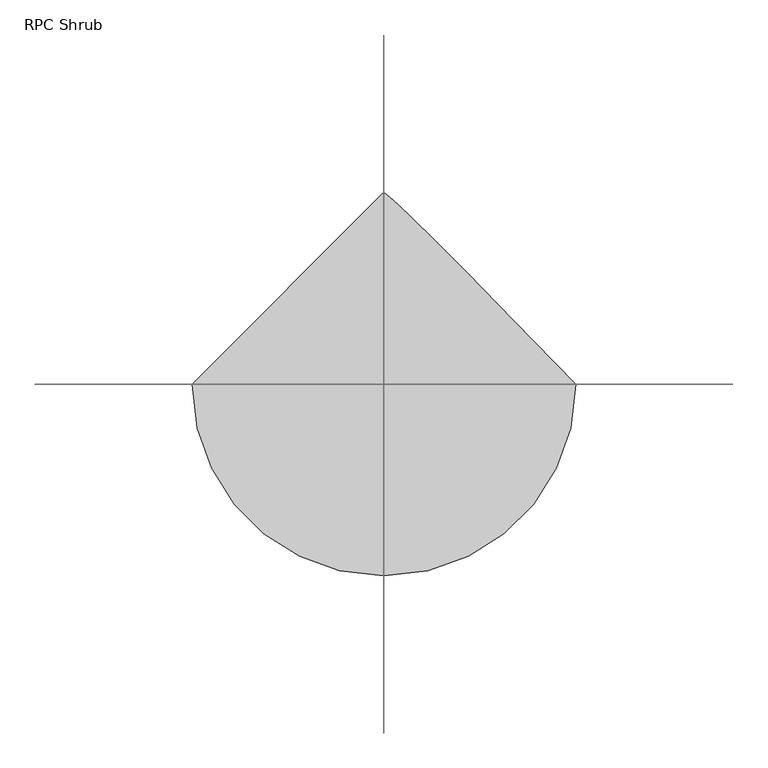
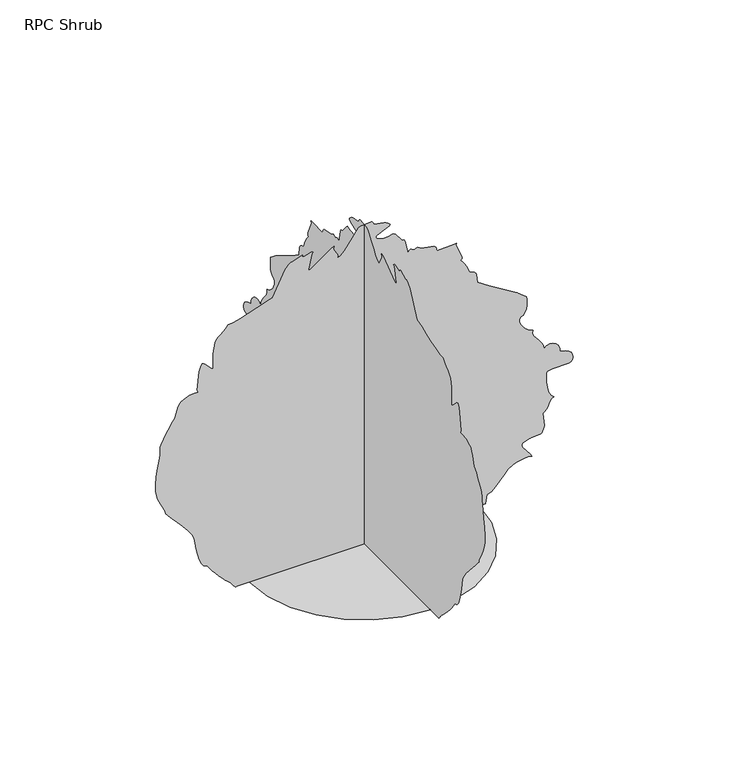
"""IFC4 building model written with IfcOpenShell, lengths in millimetres: geographic element geometry, RPC Shrub."""

from ifc_helpers import new_model, si_unit, origin, place, context, project, spatial, triangles, source, transform, mapped, element, save


def rpc_shrub_5c4a15e9(model_context):
    return source(origin(), model_context, "Body", "Tessellation", [
        triangles([(-310.4009663, 0.0, 0.0), (-302.1967432, -71.1236111, 0.0), (-278.8261857, -136.4392555, 0.0), (-242.1615087, -194.0757083, 0.0), (-194.0757083, -242.1615087, 0.0), (-136.4392555, -278.8261857, 0.0), (-71.1236111, -302.1967432, 0.0), (1.36e-05, -310.4009663, 0.0), (71.1236111, -302.1967432, 0.0), (136.4392555, -278.8261857, 0.0), (194.0757083, -242.1615087, 0.0), (242.1615087, -194.0757083, 0.0), (278.8261857, -136.4392555, 0.0), (302.1967432, -71.1236111, 0.0), (310.4009663, 2.71e-05, 0.0), (209.5283262, 103.4718092, 0.0), (134.7455816, 179.6535872, 0.0), (81.7052599, 233.0934394, 0.0), (46.0591254, 268.3410517, 0.0), (23.45852, 289.9412231, 0.0), (9.5549798, 302.4456561, 0.0), (-4.07e-05, 310.4009663, 0.0), (-352.7554667, 2.15e-05, 4.3495503), (-355.9965117, 2.13e-05, 8.4826161), (-359.0826241, 2.1e-05, 12.3234041), (-362.0188548, 2.08e-05, 15.7959676), (-364.8077834, 2.07e-05, 18.8245652), (-367.457004, 2.05e-05, 21.3332227), (-369.9665528, 2.04e-05, 23.2460988), (-375.8161594, 2.01e-05, 28.5320975), (-383.5606359, 1.96e-05, 36.3306653), (-392.4582396, 1.9e-05, 45.9079945), (-401.7775108, 1.84e-05, 56.5300297), (-410.7742001, 1.78e-05, 67.463215), (-418.7091808, 1.71e-05, 77.9737471), (-424.8483773, 1.66e-05, 87.3278091), (-434.3200376, 1.64e-05, 90.3102761), (-441.518399, 1.59e-05, 99.1873323), (-446.9133459, 1.51e-05, 112.4136326), (-450.9672046, 1.41e-05, 128.4448579), (-454.1523663, 1.31e-05, 145.7354086), (-456.9311211, 1.21e-05, 162.7404662), (-459.7733894, 1.12e-05, 177.9152122), (-465.8821009, 1.05e-05, 189.8085088), (-476.9463238, 9.6e-06, 205.0848474), (-490.9620744, 8.5e-06, 222.0754346), (-505.927767, 7.5e-06, 239.1112225), (-519.8393452, 6.6e-06, 254.5234358), (-530.6927888, 5.9e-06, 266.6443348), (-536.4840051, 5.5e-06, 273.804599), (-537.980062, 5.1e-06, 279.9056801), (-541.2769901, 4.6e-06, 287.7695352), (-545.6533945, 4.1e-06, 296.6874683), (-550.3904963, 3.6e-06, 305.9584685), (-554.7669371, 3e-06, 314.8764198), (-558.0638288, 2.6e-06, 322.7377496), (-559.5599221, 2.2e-06, 328.8413741), (-564.0633173, 1.1e-06, 346.2505222), (-564.6424607, -1e-07, 367.0963428), (-562.5393188, -1.4e-06, 389.5906094), (-558.9909525, -2.8e-06, 411.9375375), (-555.2393646, -4e-06, 432.3439227), (-552.5215799, -5e-06, 449.0164879), (-552.0770576, -5.6e-06, 460.1619922), (-551.4522048, -6.2e-06, 469.7809908), (-548.1832546, -6.8e-06, 479.8495623), (-543.0422894, -7.4e-06, 490.1772022), (-536.8090942, -8.1e-06, 500.5785295), (-530.2609838, -8.7e-06, 510.8553732), (-524.1776705, -9.2e-06, 520.822352), (-519.3338891, -9.8e-06, 530.2863819), (-514.6958364, -1.01e-05, 534.5764544), (-511.1779552, -1.05e-05, 541.7037083), (-508.3280565, -1.1e-05, 550.5352913), (-505.7042341, -1.16e-05, 559.930757), (-502.8569152, -1.21e-05, 568.7597966), (-499.3364542, -1.25e-05, 575.8870505), (-494.6984015, -1.28e-05, 580.1796301), (-488.7141738, -1.3e-05, 583.3724221), (-483.0575787, -1.32e-05, 586.1308657), (-477.4467293, -1.33e-05, 588.3914835), (-471.5996298, -1.34e-05, 590.0856388), (-465.2318499, -1.35e-05, 591.1448401), (-458.0563431, -1.35e-05, 591.5029578), (-449.7962731, -1.35e-05, 591.0940438), (-452.0898831, -1.38e-05, 597.7844058), (-446.8498687, -1.69e-05, 648.1323137), (-442.8239516, -1.75e-05, 659.7223766), (-438.0639951, -1.8e-05, 668.1551468), (-434.5155925, -1.8e-05, 667.6064884), (-430.9748566, -1.79e-05, 665.0360058), (-414.5257879, -1.68e-05, 647.428723), (-409.2578319, -1.66e-05, 644.4162615), (-408.9962199, -1.74e-05, 657.4007887), (-409.1181238, -1.79e-05, 666.2653639), (-409.3213454, -1.83e-05, 672.7017443), (-409.3035413, -1.87e-05, 678.4040852), (-408.7625133, -1.91e-05, 685.0639257), (-407.3934834, -1.96e-05, 694.3755667), (-404.8915649, -2.04e-05, 708.0306198), (-403.2913719, -2.1e-05, 717.4769182), (-399.8064829, -2.14e-05, 724.3451036), (-394.8255369, -2.17e-05, 729.6460882), (-388.7295427, -2.2e-05, 734.3907841), (-381.9096102, -2.23e-05, 739.5952629), (-374.7468206, -2.27e-05, 746.2703642), (-367.6271971, -2.33e-05, 755.4296162), (-354.5182589, -2.33e-05, 756.2449734), (-335.3386883, -2.36e-05, 761.043009), (-312.9155657, -2.4e-05, 768.2718555), (-290.0885433, -2.45e-05, 776.3821163), (-269.6872632, -2.49e-05, 783.819235), (-254.5437653, -2.53e-05, 789.0313442), (-247.4939957, -2.53e-05, 790.4715179), (-213.6794536, -2.94e-05, 858.769602), (-205.2583288, -3e-05, 869.5493946), (-197.3670409, -3.03e-05, 874.0807314), (-193.2331907, -3.03e-05, 873.8495682), (-168.7295447, -3.09e-05, 884.1188541), (-166.460806, -3.09e-05, 883.4558859), (-168.0742249, -3.06e-05, 879.0896553), (-161.877383, -3.06e-05, 879.3893463), (-144.3734641, -3.09e-05, 884.8376329), (-141.0938133, -3.09e-05, 884.1543898), (-137.9627544, -3.07e-05, 881.4086271), (-140.7920603, -3.07e-05, 880.4332506), (-150.2901451, -2.82e-05, 838.0508085), (-150.4359393, -2.79e-05, 834.0097034), (-142.0369153, -2.81e-05, 837.3624784), (-89.9201382, -3.04e-05, 875.4065952), (-81.5211142, -3.06e-05, 878.7594429), (-83.236371, -3.02e-05, 872.9860308), (-82.0336828, -2.99e-05, 867.6621552), (-72.5891921, -2.9e-05, 852.5922901), (-71.3862495, -2.87e-05, 847.2684872), (-73.1015109, -2.84e-05, 841.495075), (-63.556186, -2.86e-05, 845.6047806), (-53.0855361, -2.92e-05, 856.2092932), (-42.3674857, -3.01e-05, 870.5983858), (-32.0797166, -3.1e-05, 886.0492596), (-22.9007347, -3.19e-05, 899.8541582), (-15.50783, -3.24e-05, 909.2952971), (-10.5790577, -3.25e-05, 911.6575075), (18.9106201, -3.27e-05, 914.4007267), (21.5322068, -3.27e-05, 913.1789989), (23.8564858, -3.25e-05, 909.8845779), (26.6850082, -3.21e-05, 903.8622711), (53.36646, -3.19e-05, 899.8287237), (58.7731068, -3.17e-05, 897.4639698), (63.9669031, -3.15e-05, 893.9232702), (69.0938976, -3.12e-05, 888.8939987), (68.0601171, -3.1e-05, 885.5234196), (63.3263127, -3.08e-05, 882.1706446), (34.7215748, -3.01e-05, 870.0904226), (31.9859905, -2.99e-05, 867.6900604), (32.133565, -2.97e-05, 863.7226427), (35.5686638, -2.95e-05, 860.1538925), (41.5277613, -2.93e-05, 857.2862623), (49.2473392, -2.92e-05, 855.4244574), (57.9630999, -2.92e-05, 854.8808859), (66.9122902, -2.92e-05, 855.9553116), (75.3308715, -2.94e-05, 858.9575993), (79.5358429, -2.94e-05, 858.9905914), (84.1909094, -2.92e-05, 855.1374109), (99.0570351, -2.8e-05, 835.8054514), (103.7123468, -2.78e-05, 831.9522709), (107.9173227, -2.78e-05, 831.9827196), (110.5566329, -2.75e-05, 826.9687815), (117.7400153, -2.54e-05, 791.6018269), (122.069702, -2.57e-05, 796.2169521), (125.2845857, -2.58e-05, 797.6521116), (127.9442162, -2.57e-05, 797.0729319), (133.8415943, -2.56e-05, 794.512623), (138.1999856, -2.56e-05, 794.8580961), (144.2457012, -2.58e-05, 797.8374928), (154.0983702, -2.54e-05, 791.6500797), (188.4892397, -2.5e-05, 784.7844378), (193.5639118, -2.47e-05, 779.5723286), (196.3218285, -2.41e-05, 769.7729994), (243.3426139, -2.42e-05, 771.0379658), (249.3334547, -2.43e-05, 772.2673239), (247.7520468, -2.39e-05, 766.8596598), (263.6852313, -2.17e-05, 729.0644377), (264.3888039, -2.13e-05, 722.3968941), (260.2486133, -2.11e-05, 719.5673429), (264.4396183, -2.09e-05, 715.6404751), (268.5899827, -2.05e-05, 710.080422), (272.58794, -2.02e-05, 703.4306826), (276.3268288, -1.97e-05, 696.2399878), (279.6948645, -1.93e-05, 689.0492203), (282.5828423, -1.89e-05, 682.4020243), (284.8815392, -1.86e-05, 676.8470581), (292.1535699, -1.84e-05, 674.5203833), (297.5205933, -1.82e-05, 671.6629269), (301.2772681, -1.8e-05, 668.0231054), (303.7181983, -1.78e-05, 663.3520243), (306.0880391, -1.64e-05, 640.6748474), (337.5484735, -1.51e-05, 619.285528), (412.8366832, -1.23e-05, 572.7882208), (438.1198783, -1.12e-05, 553.4791523), (439.8826341, -1.08e-05, 546.9589471), (439.9893136, -9.7e-06, 528.3128105), (438.1224217, -9.1e-06, 518.4956772), (434.833124, -8.6e-06, 509.8850836), (430.0172479, -8.2e-06, 503.634157), (423.57073, -8.1e-06, 500.8960247), (419.6083265, -7.7e-06, 495.2673712), (419.9613936, -7.3e-06, 487.2053996), (423.7561475, -6.7e-06, 477.8835849), (430.1112465, -6.1e-06, 468.4703513), (438.1503633, -5.6e-06, 460.136594), (446.9946273, -5.3e-06, 454.0533171), (455.7652765, -5.1e-06, 451.3913793), (454.5663671, -4.6e-06, 443.4767461), (457.9420332, -4.1e-06, 435.1353584), (464.2260246, -3.6e-06, 426.3952306), (471.7495116, -3.1e-06, 417.2791446), (478.8462805, -2.5e-06, 407.8151147), (483.8449943, -1.9e-06, 398.025923), (485.0794393, -1.3e-06, 387.9344968), (492.6181506, -1.7e-06, 394.3632468), (501.3405107, -1.8e-06, 396.5095548), (510.2914905, -1.8e-06, 394.9982735), (518.5109379, -1.5e-06, 390.4541831), (525.0463675, -1.1e-06, 383.5047526), (528.9401705, -5e-07, 374.7773057), (529.2322675, 0.0, 364.8966951), (543.28359, 2e-07, 361.6200783), (553.2505325, 5e-07, 356.9591709), (559.7300789, 8e-07, 351.3864369), (563.3267344, 1.2e-06, 345.3742312), (564.6424607, 1.5e-06, 339.3975975), (564.2741693, 1.9e-06, 333.9264562), (562.8263652, 2.1e-06, 329.438249), (558.5058077, 2.4e-06, 325.0237292), (551.6808246, 2.5e-06, 323.3371679), (508.3052018, 2.5e-06, 323.4667022), (495.6814084, 2.7e-06, 320.1113837), (493.0550426, 3e-06, 315.2853702), (491.9247336, 3.6e-06, 304.683401), (492.3870237, 4.5e-06, 290.5000371), (494.5434691, 5.4e-06, 274.934908), (498.4855614, 6.3e-06, 260.1850997), (504.3148567, 7e-06, 248.4462268), (512.1304407, 7.4e-06, 241.918682), (506.1944658, 7.6e-06, 237.9293542), (502.0110729, 7.9e-06, 232.375896), (498.8894248, 8.3e-06, 225.9143899), (496.1360682, 8.7e-06, 219.2011551), (493.06518, 9.1e-06, 212.8918018), (488.9859595, 9.4e-06, 207.6423766), (483.2074605, 9.6e-06, 204.1089804), (486.5094392, 1.18e-05, 167.9235982), (484.7949363, 1.23e-05, 159.1671923), (479.7174846, 1.29e-05, 149.4257811), (478.0410971, 1.3e-05, 147.3986065), (448.2189348, 1.31e-05, 145.3638107), (427.0784738, 1.35e-05, 138.6241693), (425.673872, 1.39e-05, 132.82763), (427.5890167, 1.42e-05, 126.7778539), (449.1968184, 1.58e-05, 99.5421708), (453.2709884, 1.63e-05, 91.8492719), (446.9844898, 1.62e-05, 94.1108889), (432.729982, 1.62e-05, 94.2706539), (416.3113984, 1.64e-05, 90.1472137), (414.6045259, 1.65e-05, 89.3547294), (401.3177642, 1.66e-05, 85.9130245), (388.9555827, 1.72e-05, 76.9775597), (377.2588766, 1.79e-05, 64.7009653), (365.9660339, 1.87e-05, 51.235649), (354.8103559, 1.95e-05, 38.7350312), (343.5327375, 2e-05, 29.3512471), (331.8716034, 2.03e-05, 25.2371292), (326.9541347, 2.18e-05, 4e-05), (-349.3544025, 2.18e-05, 4e-05), (-4.6e-06, -352.7554667, 4.3495758), (-4.6e-06, -355.9965117, 8.4826416), (-4.6e-06, -359.0826241, 12.3234041), (-4.6e-06, -362.0188548, 15.7959937), (-4.6e-06, -364.8077834, 18.8245902), (-4.6e-06, -367.457004, 21.3332477), (-4.6e-06, -369.9665528, 23.2460988), (-4.6e-06, -375.8161594, 28.5320975), (-4.6e-06, -383.5606359, 36.3306653), (-4.6e-06, -392.4582396, 45.9079945), (-4.6e-06, -401.7775108, 56.5300297), (-4.6e-06, -410.7742001, 67.4634693), (-4.6e-06, -418.7091808, 77.9737471), (-4.6e-06, -424.8483773, 87.3278091), (-4.6e-06, -434.3200376, 90.3102761), (-4.6e-06, -441.518399, 99.1873323), (-4.6e-06, -446.9133459, 112.4138869), (-4.6e-06, -450.9672046, 128.4448579), (-4.6e-06, -454.1523663, 145.7354086), (-4.6e-06, -456.9311211, 162.7404662), (-4.6e-06, -459.7733894, 177.9152122), (-4.6e-06, -465.8821009, 189.8085088), (-4.6e-06, -476.9463238, 205.0848474), (-4.6e-06, -490.9620744, 222.0754346), (-4.6e-06, -505.927767, 239.1112225), (-4.6e-06, -519.8393452, 254.5234358), (-4.6e-06, -530.6927888, 266.6443348), (-4.6e-06, -536.4840051, 273.804599), (-4.6e-06, -537.980062, 279.9056801), (-4.6e-06, -541.2769901, 287.7695352), (-4.6e-06, -545.6533945, 296.6874683), (-4.6e-06, -550.3904963, 305.9584685), (-4.6e-06, -554.7669371, 314.8764198), (-4.6e-06, -558.0638288, 322.7377496), (-4.6e-06, -559.5599221, 328.8413741), (-4.6e-06, -564.0633173, 346.2505222), (-4.6e-06, -564.6424607, 367.0963428), (-4.6e-06, -562.5393188, 389.5906094), (-4.6e-06, -558.9909525, 411.9375375), (-4.6e-06, -555.2393646, 432.3439227), (-4.6e-06, -552.5215799, 449.0164879), (-4.6e-06, -552.0770576, 460.1619922), (-4.6e-06, -551.4522048, 469.7809908), (-4.6e-06, -548.1832546, 479.8495623), (-4.6e-06, -543.0422894, 490.1772022), (-4.6e-06, -536.8090942, 500.5785295), (-4.6e-06, -530.2609838, 510.8553732), (-4.6e-06, -524.1776705, 520.822352), (-4.6e-06, -519.3338891, 530.2863819), (-4.6e-06, -514.6958364, 534.5764544), (-4.6e-06, -511.1779552, 541.7037083), (-4.6e-06, -508.3280565, 550.5352913), (-4.6e-06, -505.7042341, 559.930757), (-4.6e-06, -502.8569152, 568.7597966), (-4.6e-06, -499.3364542, 575.889594), (-4.6e-06, -494.6984015, 580.1796301), (-4.6e-06, -488.7141738, 583.3724221), (-4.6e-06, -483.0575787, 586.1308657), (-4.6e-06, -477.4467293, 588.3914835), (-4.6e-06, -471.5996298, 590.0856388), (-4.6e-06, -465.2318499, 591.1448401), (-4.6e-06, -458.0563431, 591.5029578), (-4.6e-06, -449.7962731, 591.0940438), (-4.6e-06, -452.0898831, 597.7844058), (-4.6e-06, -446.8498687, 648.1323137), (-4.6e-06, -442.8239516, 659.7223766), (-4.6e-06, -438.0639951, 668.1551468), (-4.6e-06, -434.5155925, 667.6064884), (-4.6e-06, -430.9748566, 665.0360058), (-4.6e-06, -414.5257879, 647.428723), (-4.6e-06, -409.2578319, 644.4162615), (-4.6e-06, -408.9962199, 657.4007887), (-4.6e-06, -409.1181238, 666.2653639), (-4.6e-06, -409.3213454, 672.7017443), (-4.6e-06, -409.3035413, 678.4040852), (-4.6e-06, -408.7625133, 685.0639257), (-4.6e-06, -407.3934834, 694.3755667), (-4.6e-06, -404.8915649, 708.0306198), (-4.6e-06, -403.2913719, 717.4769182), (-4.6e-06, -399.8064829, 724.3451036), (-4.6e-06, -394.8255369, 729.6460882), (-4.6e-06, -388.7295427, 734.3907841), (-4.6e-06, -381.9096102, 739.5952629), (-4.6e-06, -374.7468206, 746.2703642), (-4.6e-06, -367.6271971, 755.4296162), (-4.6e-06, -354.5182589, 756.2449734), (-4.6e-06, -335.3386883, 761.043009), (-4.6e-06, -312.9155657, 768.2718555), (-4.6e-06, -290.0885433, 776.3821163), (-4.6e-06, -269.6872632, 783.819235), (-4.6e-06, -254.5437653, 789.0313442), (-4.6e-06, -247.4939957, 790.4715179), (-4.6e-06, -213.6794536, 858.769602), (-4.6e-06, -205.2583288, 869.5493946), (-4.6e-06, -197.3670409, 874.0807314), (-4.6e-06, -193.2331907, 873.8495682), (-4.6e-06, -168.7295447, 884.1188541), (-4.6e-06, -166.4605516, 883.4558859), (-4.6e-06, -168.0742249, 879.0896553), (-4.6e-06, -161.877383, 879.3893463), (-4.6e-06, -144.3734641, 884.8376329), (-4.6e-06, -141.0938133, 884.1543898), (-4.6e-06, -137.9627544, 881.4086271), (-4.6e-06, -140.7920603, 880.4332506), (-4.6e-06, -150.2901451, 838.0508085), (-4.6e-06, -150.4359393, 834.0121742), (-4.6e-06, -142.0369153, 837.3624784), (-4.6e-06, -89.9201382, 875.4065952), (-4.6e-06, -81.5211142, 878.7594429), (-4.6e-06, -83.236371, 872.9860308), (-4.6e-06, -82.0336828, 867.6621552), (-4.6e-06, -72.5891921, 852.5922901), (-4.6e-06, -71.3862495, 847.2684872), (-4.6e-06, -73.1015109, 841.495075), (-4.6e-06, -63.556186, 845.6047806), (-4.6e-06, -53.0855361, 856.2092932), (-4.6e-06, -42.3674857, 870.5983858), (-4.6e-06, -32.0797166, 886.0492596), (-4.6e-06, -22.9007347, 899.8541582), (-4.6e-06, -15.50783, 909.2952971), (-4.6e-06, -10.5790577, 911.6575075), (-4.6e-06, 18.9106201, 914.4007267), (-4.6e-06, 21.5322068, 913.1789989), (-4.6e-06, 23.8564858, 909.8845779), (-4.6e-06, 26.6850082, 903.8622711), (-4.6e-06, 53.36646, 899.8287237), (-4.6e-06, 58.7731068, 897.4639698), (-4.6e-06, 63.9669031, 893.9232702), (-4.6e-06, 69.0938976, 888.8939987), (-4.6e-06, 68.0601171, 885.5234196), (-4.6e-06, 63.3263127, 882.173188), (-4.6e-06, 34.7215748, 870.0904226), (-4.6e-06, 31.9859905, 867.6900604), (-4.6e-06, 32.133565, 863.7226427), (-4.6e-06, 35.5686638, 860.1538925), (-4.6e-06, 41.5277613, 857.2862623), (-4.6e-06, 49.2473392, 855.4269281), (-4.6e-06, 57.9630999, 854.8808859), (-4.6e-06, 66.9122902, 855.9553116), (-4.6e-06, 75.3308715, 858.9575993), (-4.6e-06, 79.5358429, 858.9905914), (-4.6e-06, 84.1909094, 855.1374109), (-4.6e-06, 99.0570351, 835.8054514), (-4.6e-06, 103.7123468, 831.9522709), (-4.6e-06, 107.9173227, 831.9852631), (-4.6e-06, 110.5566329, 826.9687815), (-4.6e-06, 117.7400153, 791.6018269), (-4.6e-06, 122.069702, 796.2169521), (-4.6e-06, 125.2845857, 797.6521116), (-4.6e-06, 127.9442162, 797.0729319), (-4.6e-06, 133.8415943, 794.512623), (-4.6e-06, 138.1999856, 794.8580961), (-4.6e-06, 144.2457012, 797.8374928), (-4.6e-06, 154.0983702, 791.6500797), (-4.6e-06, 188.4892397, 784.7844378), (-4.6e-06, 193.5639118, 779.5723286), (-4.6e-06, 196.3218285, 769.7729994), (-4.6e-06, 243.3426139, 771.0379658), (-4.6e-06, 249.3334547, 772.2673239), (-4.6e-06, 247.7520468, 766.8596598), (-4.6e-06, 263.6852313, 729.0644377), (-4.6e-06, 264.3888039, 722.3968941), (-4.6e-06, 260.2486133, 719.5673429), (-4.6e-06, 264.4396183, 715.6404751), (-4.6e-06, 268.5899827, 710.080422), (-4.6e-06, 272.58794, 703.4306826), (-4.6e-06, 276.3268288, 696.2399878), (-4.6e-06, 279.6948645, 689.0492203), (-4.6e-06, 282.5828423, 682.4020243), (-4.6e-06, 284.8815392, 676.8470581), (-4.6e-06, 292.1535699, 674.5203833), (-4.6e-06, 297.5205933, 671.6629269), (-4.6e-06, 301.2772681, 668.0231054), (-4.6e-06, 303.7181983, 663.3520243), (-4.6e-06, 306.0880391, 640.6748474), (-4.6e-06, 337.5484735, 619.285528), (-4.6e-06, 412.8366832, 572.7907642), (-4.6e-06, 438.1198783, 553.4791523), (-4.6e-06, 439.8826341, 546.9589471), (-4.6e-06, 439.9893136, 528.3128105), (-4.6e-06, 438.1224217, 518.4956772), (-4.6e-06, 434.833124, 509.8850836), (-4.6e-06, 430.0172479, 503.634157), (-4.6e-06, 423.57073, 500.8960247), (-4.6e-06, 419.6083265, 495.2673712), (-4.6e-06, 419.9613936, 487.2053996), (-4.6e-06, 423.7561475, 477.8835849), (-4.6e-06, 430.1112465, 468.4703513), (-4.6e-06, 438.1503633, 460.136594), (-4.6e-06, 446.9946273, 454.0533171), (-4.6e-06, 455.7652765, 451.3913793), (-4.6e-06, 454.5663671, 443.4767461), (-4.6e-06, 457.9420332, 435.1353584), (-4.6e-06, 464.2260246, 426.3952306), (-4.6e-06, 471.7495116, 417.2791446), (-4.6e-06, 478.8462805, 407.8151147), (-4.6e-06, 483.8449943, 398.025923), (-4.6e-06, 485.0794393, 387.9344968), (-4.6e-06, 492.6181506, 394.3632468), (-4.6e-06, 501.3405107, 396.5095548), (-4.6e-06, 510.2914905, 394.9982735), (-4.6e-06, 518.5109379, 390.4541831), (-4.6e-06, 525.0463675, 383.5047526), (-4.6e-06, 528.9401705, 374.7773057), (-4.6e-06, 529.2322675, 364.8966951), (-4.6e-06, 543.28359, 361.6200783), (-4.6e-06, 553.2505325, 356.9591709), (-4.6e-06, 559.7300789, 351.3864369), (-4.6e-06, 563.3267344, 345.3742312), (-4.6e-06, 564.6424607, 339.3975975), (-4.6e-06, 564.2741693, 333.9264562), (-4.6e-06, 562.8263652, 329.438249), (-4.6e-06, 558.5058077, 325.0237292), (-4.6e-06, 551.6808246, 323.3371679), (-4.6e-06, 508.3052018, 323.4667022), (-4.6e-06, 495.6814084, 320.1113837), (-4.6e-06, 493.0550426, 315.2853702), (-4.6e-06, 491.9247336, 304.683401), (-4.6e-06, 492.3870237, 290.5000371), (-4.6e-06, 494.5434691, 274.934908), (-4.6e-06, 498.4855614, 260.1850997), (-4.6e-06, 504.3148567, 248.4464812), (-4.6e-06, 512.1304407, 241.918682), (-4.6e-06, 506.1944658, 237.9293542), (-4.6e-06, 502.0110729, 232.375896), (-4.6e-06, 498.8894248, 225.9143899), (-4.6e-06, 496.1360682, 219.2011551), (-4.6e-06, 493.06518, 212.8918018), (-4.6e-06, 488.9859595, 207.6423766), (-4.6e-06, 483.2074605, 204.1089804), (-4.6e-06, 486.5094392, 167.9235982), (-4.6e-06, 484.7949363, 159.1671923), (-4.6e-06, 479.7174846, 149.4257811), (-4.6e-06, 478.0410971, 147.3988609), (-4.6e-06, 448.2189348, 145.3638107), (-4.6e-06, 427.0784738, 138.6241693), (-4.6e-06, 425.673872, 132.8278843), (-4.6e-06, 427.5890167, 126.7778539), (-4.6e-06, 449.1968184, 99.5421708), (-4.6e-06, 453.2709884, 91.8492719), (-4.6e-06, 446.9844898, 94.1108889), (-4.6e-06, 432.729982, 94.2706539), (-4.6e-06, 416.3113984, 90.1472137), (-4.6e-06, 414.6045259, 89.3547294), (-4.6e-06, 401.3177642, 85.9130245), (-4.6e-06, 388.9555827, 76.9775597), (-4.6e-06, 377.2588766, 64.7009653), (-4.6e-06, 365.9660339, 51.235649), (-4.6e-06, 354.8103559, 38.7350312), (-4.6e-06, 343.5327375, 29.3512471), (-4.6e-06, 331.8716034, 25.2371564), (-4.6e-06, 326.9541347, 6.03e-05), (-4.6e-06, -349.3544025, 6.03e-05)], [[21, 22, 1], [20, 21, 1], [19, 20, 1], [18, 19, 1], [17, 18, 1], [17, 1, 2], [17, 2, 3], [17, 3, 4], [16, 17, 4], [16, 4, 5], [16, 5, 6], [16, 6, 7], [16, 7, 8], [16, 8, 9], [16, 9, 10], [16, 10, 11], [16, 11, 12], [15, 16, 12], [14, 15, 12], [13, 14, 12], [261, 262, 263], [130, 131, 132], [124, 125, 126], [180, 181, 182], [244, 245, 246], [119, 120, 121], [118, 119, 121], [212, 213, 214], [273, 274, 275], [123, 124, 126], [260, 261, 263], [88, 89, 90], [88, 90, 91], [260, 263, 264], [87, 88, 91], [87, 91, 92], [122, 123, 126], [166, 167, 168], [150, 151, 152], [150, 152, 153], [149, 150, 153], [148, 149, 153], [148, 153, 154], [147, 148, 154], [147, 154, 155], [87, 92, 93], [183, 184, 185], [122, 126, 127], [121, 122, 127], [174, 175, 176], [130, 132, 133], [129, 130, 133], [260, 264, 265], [129, 133, 134], [129, 134, 135], [129, 135, 136], [273, 275, 23], [86, 87, 93], [85, 86, 93], [273, 23, 24], [273, 24, 25], [273, 25, 26], [118, 121, 127], [118, 127, 128], [106, 107, 108], [273, 26, 27], [260, 265, 266], [260, 266, 267], [259, 260, 267], [244, 246, 247], [179, 180, 182], [273, 27, 28], [255, 256, 257], [162, 163, 164], [161, 162, 164], [117, 118, 128], [116, 117, 128], [115, 116, 128], [114, 115, 128], [273, 28, 29], [273, 29, 30], [273, 30, 31], [273, 31, 32], [273, 32, 33], [273, 33, 34], [273, 34, 35], [273, 35, 36], [161, 164, 165], [170, 171, 172], [169, 170, 172], [169, 172, 173], [254, 255, 257], [253, 254, 257], [252, 253, 257], [252, 257, 258], [243, 244, 247], [160, 161, 165], [36, 37, 38], [243, 247, 248], [36, 38, 39], [273, 36, 39], [273, 39, 40], [273, 40, 41], [273, 41, 42], [273, 42, 43], [273, 43, 44], [273, 44, 45], [273, 45, 46], [273, 46, 47], [272, 273, 47], [271, 272, 47], [270, 271, 47], [269, 270, 47], [268, 269, 47], [267, 268, 47], [259, 267, 47], [258, 259, 47], [252, 258, 47], [252, 47, 48], [252, 48, 49], [252, 49, 50], [252, 50, 51], [252, 51, 52], [252, 52, 53], [252, 53, 54], [252, 54, 55], [252, 55, 56], [252, 56, 57], [252, 57, 58], [252, 58, 59], [252, 59, 60], [252, 60, 61], [252, 61, 62], [252, 62, 63], [252, 63, 64], [252, 64, 65], [252, 65, 66], [252, 66, 67], [252, 67, 68], [252, 68, 69], [252, 69, 70], [252, 70, 71], [252, 71, 72], [252, 72, 73], [252, 73, 74], [252, 74, 75], [252, 75, 76], [252, 76, 77], [252, 77, 78], [252, 78, 79], [252, 79, 80], [252, 80, 81], [252, 81, 82], [252, 82, 83], [252, 83, 84], [252, 84, 85], [252, 85, 93], [252, 93, 94], [252, 94, 95], [252, 95, 96], [252, 96, 97], [252, 97, 98], [252, 98, 99], [252, 99, 100], [252, 100, 101], [252, 101, 102], [252, 102, 103], [252, 103, 104], [252, 104, 105], [252, 105, 106], [252, 106, 108], [252, 108, 109], [252, 109, 110], [252, 110, 111], [252, 111, 112], [252, 112, 113], [252, 113, 114], [252, 114, 128], [252, 128, 129], [252, 129, 136], [252, 136, 137], [252, 137, 138], [251, 252, 138], [250, 251, 138], [249, 250, 138], [248, 249, 138], [243, 248, 138], [242, 243, 138], [241, 242, 138], [240, 241, 138], [239, 240, 138], [238, 239, 138], [238, 138, 139], [238, 139, 140], [238, 140, 141], [238, 141, 142], [238, 142, 143], [237, 238, 143], [234, 235, 236], [233, 234, 236], [232, 233, 236], [231, 232, 236], [230, 231, 236], [229, 230, 236], [228, 229, 236], [227, 228, 236], [227, 236, 237], [179, 182, 183], [179, 183, 185], [199, 200, 201], [199, 201, 202], [199, 202, 203], [199, 203, 204], [199, 204, 205], [199, 205, 206], [199, 206, 207], [198, 199, 207], [198, 207, 208], [144, 145, 146], [144, 146, 147], [144, 147, 155], [143, 144, 155], [143, 155, 156], [237, 143, 156], [237, 156, 157], [237, 157, 158], [237, 158, 159], [237, 159, 160], [177, 178, 179], [226, 227, 237], [225, 226, 237], [224, 225, 237], [223, 224, 237], [222, 223, 237], [221, 222, 237], [220, 221, 237], [220, 237, 160], [219, 220, 160], [218, 219, 160], [166, 168, 169], [165, 166, 169], [160, 165, 169], [218, 160, 169], [217, 218, 169], [216, 217, 169], [215, 216, 169], [215, 169, 173], [215, 173, 174], [215, 174, 176], [211, 212, 214], [211, 214, 215], [194, 195, 196], [193, 194, 196], [192, 193, 196], [192, 196, 197], [197, 198, 208], [176, 177, 179], [197, 208, 209], [176, 179, 185], [185, 186, 187], [176, 185, 187], [176, 187, 188], [176, 188, 189], [176, 189, 190], [176, 190, 191], [176, 191, 192], [176, 192, 197], [176, 197, 209], [176, 209, 210], [215, 176, 210], [211, 215, 210], [514, 515, 516], [383, 384, 385], [377, 378, 379], [433, 434, 435], [497, 498, 499], [372, 373, 374], [371, 372, 374], [465, 466, 467], [526, 527, 528], [376, 377, 379], [513, 514, 516], [341, 342, 343], [341, 343, 344], [513, 516, 517], [340, 341, 344], [340, 344, 345], [375, 376, 379], [419, 420, 421], [403, 404, 405], [403, 405, 406], [402, 403, 406], [401, 402, 406], [401, 406, 407], [400, 401, 407], [400, 407, 408], [340, 345, 346], [436, 437, 438], [375, 379, 380], [374, 375, 380], [427, 428, 429], [383, 385, 386], [382, 383, 386], [513, 517, 518], [382, 386, 387], [382, 387, 388], [382, 388, 389], [526, 528, 276], [339, 340, 346], [338, 339, 346], [526, 276, 277], [526, 277, 278], [526, 278, 279], [371, 374, 380], [371, 380, 381], [359, 360, 361], [526, 279, 280], [513, 518, 519], [513, 519, 520], [512, 513, 520], [497, 499, 500], [432, 433, 435], [526, 280, 281], [508, 509, 510], [415, 416, 417], [414, 415, 417], [370, 371, 381], [369, 370, 381], [368, 369, 381], [367, 368, 381], [526, 281, 282], [526, 282, 283], [526, 283, 284], [526, 284, 285], [526, 285, 286], [526, 286, 287], [526, 287, 288], [526, 288, 289], [414, 417, 418], [423, 424, 425], [422, 423, 425], [422, 425, 426], [507, 508, 510], [506, 507, 510], [505, 506, 510], [505, 510, 511], [496, 497, 500], [413, 414, 418], [289, 290, 291], [496, 500, 501], [289, 291, 292], [526, 289, 292], [526, 292, 293], [526, 293, 294], [526, 294, 295], [526, 295, 296], [526, 296, 297], [526, 297, 298], [526, 298, 299], [526, 299, 300], [525, 526, 300], [524, 525, 300], [523, 524, 300], [522, 523, 300], [521, 522, 300], [520, 521, 300], [512, 520, 300], [511, 512, 300], [505, 511, 300], [505, 300, 301], [505, 301, 302], [505, 302, 303], [505, 303, 304], [505, 304, 305], [505, 305, 306], [505, 306, 307], [505, 307, 308], [505, 308, 309], [505, 309, 310], [505, 310, 311], [505, 311, 312], [505, 312, 313], [505, 313, 314], [505, 314, 315], [505, 315, 316], [505, 316, 317], [505, 317, 318], [505, 318, 319], [505, 319, 320], [505, 320, 321], [505, 321, 322], [505, 322, 323], [505, 323, 324], [505, 324, 325], [505, 325, 326], [505, 326, 327], [505, 327, 328], [505, 328, 329], [505, 329, 330], [505, 330, 331], [505, 331, 332], [505, 332, 333], [505, 333, 334], [505, 334, 335], [505, 335, 336], [505, 336, 337], [505, 337, 338], [505, 338, 346], [505, 346, 347], [505, 347, 348], [505, 348, 349], [505, 349, 350], [505, 350, 351], [505, 351, 352], [505, 352, 353], [505, 353, 354], [505, 354, 355], [505, 355, 356], [505, 356, 357], [505, 357, 358], [505, 358, 359], [505, 359, 361], [505, 361, 362], [505, 362, 363], [505, 363, 364], [505, 364, 365], [505, 365, 366], [505, 366, 367], [505, 367, 381], [505, 381, 382], [505, 382, 389], [505, 389, 390], [505, 390, 391], [504, 505, 391], [503, 504, 391], [502, 503, 391], [501, 502, 391], [496, 501, 391], [495, 496, 391], [494, 495, 391], [493, 494, 391], [492, 493, 391], [491, 492, 391], [491, 391, 392], [491, 392, 393], [491, 393, 394], [491, 394, 395], [491, 395, 396], [490, 491, 396], [487, 488, 489], [486, 487, 489], [485, 486, 489], [484, 485, 489], [483, 484, 489], [482, 483, 489], [481, 482, 489], [480, 481, 489], [480, 489, 490], [432, 435, 436], [432, 436, 438], [452, 453, 454], [452, 454, 455], [452, 455, 456], [452, 456, 457], [452, 457, 458], [452, 458, 459], [452, 459, 460], [451, 452, 460], [451, 460, 461], [397, 398, 399], [397, 399, 400], [397, 400, 408], [396, 397, 408], [396, 408, 409], [490, 396, 409], [490, 409, 410], [490, 410, 411], [490, 411, 412], [490, 412, 413], [430, 431, 432], [479, 480, 490], [478, 479, 490], [477, 478, 490], [476, 477, 490], [475, 476, 490], [474, 475, 490], [473, 474, 490], [473, 490, 413], [472, 473, 413], [471, 472, 413], [419, 421, 422], [418, 419, 422], [413, 418, 422], [471, 413, 422], [470, 471, 422], [469, 470, 422], [468, 469, 422], [468, 422, 426], [468, 426, 427], [468, 427, 429], [464, 465, 467], [464, 467, 468], [447, 448, 449], [446, 447, 449], [445, 446, 449], [445, 449, 450], [450, 451, 461], [429, 430, 432], [450, 461, 462], [429, 432, 438], [438, 439, 440], [429, 438, 440], [429, 440, 441], [429, 441, 442], [429, 442, 443], [429, 443, 444], [429, 444, 445], [429, 445, 450], [429, 450, 462], [429, 462, 463], [468, 429, 463], [464, 468, 463]], closed=False),
    ])


if __name__ == "__main__":
    model = new_model("IFC4")
    model_context = context("Model", 3, world=origin())
    ifc_project = project(units=[si_unit("LENGTHUNIT", "METRE", prefix="MILLI")], contexts=[model_context])
    site = spatial("IfcSite", under=ifc_project)
    building = spatial("IfcBuilding", under=site)
    placement = place(None, origin())
    rpc_shrub_shape = rpc_shrub_5c4a15e9(model_context)
    element("IfcGeographicElement", 1, ObjectType="RPC Shrub : Vibernum 3'-0\"", at=placement, inside=building, context=model_context, shape_type="MappedRepresentation", body=[
        mapped(rpc_shrub_shape, transform((0.0, 0.0, 0.0), x_axis=(1.0, 0.0, 0.0), y_axis=(0.0, 1.0, 0.0), z_axis=(0.0, 0.0, 1.0))),
    ])
    save(model, "model.ifc")

# Revit data of these elements
# Type "RPC Shrub : Vibernum 3'-0\""
#   Type Comments = "Vibernum"
#   built-in parameter 1005198 = "{2, 15},{39, RPC-16-FU5P-8RFX-7Q0N-4000-ST1L-LVER-AU},{1, 0},{1, 0},{2, 13},{1, 8},{5, Color},{1, 0},{1, 0},{3, 0.8},{3, 0.8},{3, 0.8},{1, 8},{7, BBoxMin},{1, 0},{1, 0},{1, 0},{1, 0},{1, 0},{1, 8},{7, BBoxMax},{1, 0},{1, 0},{1, 0},{1, 0},{1, 0},{2, 11},{9, RPCTypeId},{1, 0},{1, 0},{39, RPC-16-FU5P-8RFX-7Q0N-4000-ST1L-LVER-AU},{1, 6},{14, RPCPlantHeight},{1, 0},{1, 0},{1, 3},{2, 11},{7, keyword},{1, 0},{1, 0},{35, :RPCs:Shrubs & Grasses:Geometry:RPC},{2, 11},{8, category},{1, 0},{1, 0},{16, Shrubs & Grasses},{2, 11},{12, LocalizedUID},{1, 0},{1, 0},{8, Vibernum},{2, 14},{6, Height},{1, 0},{1, 0},{1, 3},{1, 2},{16, Cast Reflections},{1, 0},{1, 0},{1, 0},{1, 2},{12, Cast Shadows},{1, 0},{1, 0},{1, 1},{1, 2},{9, Lock View},{1, 0},{1, 0},{1, 0},{1, 4},{5, ViewC},{1, 0},{1, 0},{1, 0},{21, assetlibrary_base.fbx},{1, 5},"
#   built-in parameter 1005195 = "RPC-16-FU5P-8RFX-7Q0N-4000-ST1L-LVER-AU"
#   Assembly Code = "G2050500"
#   Height = 3' - 0"
#   Default Elevation = 0
